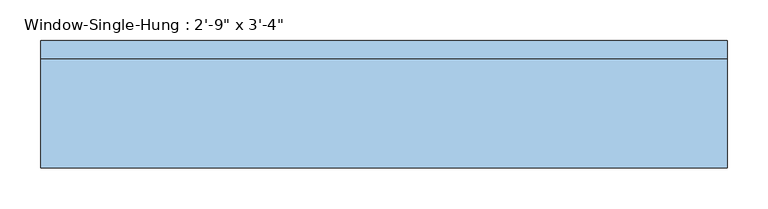
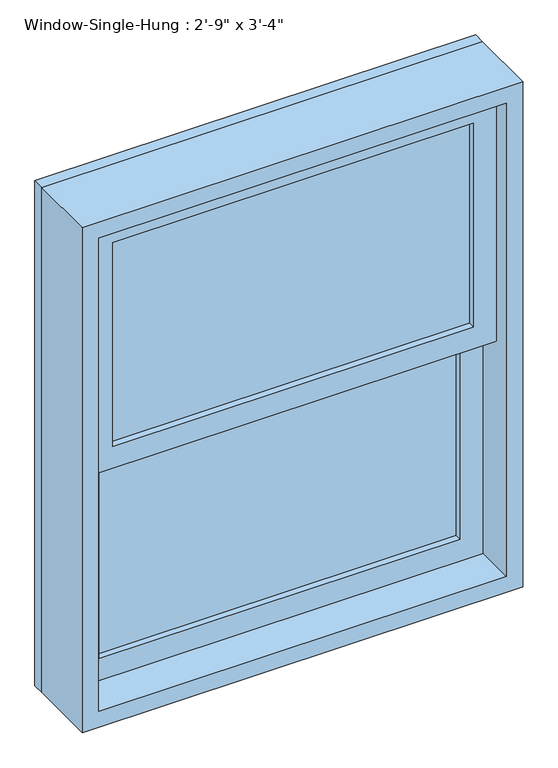
"""IFC4 building model written with IfcOpenShell, lengths in millimetres: window geometry."""

from ifc_helpers import new_model, si_unit, frame, origin, place, context, project, spatial, polyline, outline, extrude, source, transform, mapped, element, save


def window_d23c6517(model_context):
    return source(origin(), model_context, "Body", "SweptSolid", [
        extrude(outline(polyline([(342.9, 1.5875), (-342.9, 1.5875), (-342.9, 7.9375), (342.9, 7.9375), (342.9, 1.5875)])), frame((0.0, 0.0, 990.6), z_axis=(0.0, 0.0, 1.0), x_axis=(1.0, 0.0, 0.0)), (0.0, 0.0, 1.0), 409.575),
        extrude(outline(polyline([(-342.9, 14.2875), (-342.9, 20.6375), (342.9, 20.6375), (342.9, 14.2875), (-342.9, 14.2875)])), frame((0.0, 0.0, 990.6), z_axis=(0.0, 0.0, 1.0), x_axis=(1.0, 0.0, 0.0)), (0.0, 0.0, 1.0), 409.575),
        extrude(outline(polyline([(342.9, -42.8625), (-342.9, -42.8625), (-342.9, -36.5125), (342.9, -36.5125), (342.9, -42.8625)])), frame((0.0, 0.0, 1444.625), z_axis=(0.0, 0.0, 1.0), x_axis=(1.0, 0.0, 0.0)), (0.0, 0.0, 1.0), 409.575),
        extrude(outline(polyline([(-342.9, -30.1625), (-342.9, -23.8125), (342.9, -23.8125), (342.9, -30.1625), (-342.9, -30.1625)])), frame((0.0, 0.0, 1444.625), z_axis=(0.0, 0.0, 1.0), x_axis=(1.0, 0.0, 0.0)), (0.0, 0.0, 1.0), 409.575),
        extrude(outline(polyline([(1444.625, 387.35), (1444.625, -387.35), (946.15, -387.35), (946.15, 387.35), (1444.625, 387.35)]), holes=[polyline([(1400.175, -342.9), (1400.175, 342.9), (990.6, 342.9), (990.6, -342.9), (1400.175, -342.9)])]), frame((0.0, -11.1125, 0.0), z_axis=(0.0, 1.0, 0.0), x_axis=(0.0, 0.0, 1.0)), (0.0, 0.0, 1.0), 44.45),
        extrude(outline(polyline([(1898.65, 387.35), (1898.65, -387.35), (1400.175, -387.35), (1400.175, 387.35), (1898.65, 387.35)]), holes=[polyline([(1854.2, -342.9), (1854.2, 342.9), (1444.625, 342.9), (1444.625, -342.9), (1854.2, -342.9)])]), frame((0.0, -55.5625, 0.0), z_axis=(0.0, 1.0, 0.0), x_axis=(0.0, 0.0, 1.0)), (0.0, 0.0, 1.0), 44.45),
        extrude(outline(polyline([(1930.4, 419.1), (1930.4, -419.1), (914.4, -419.1), (914.4, 419.1), (1930.4, 419.1)]), holes=[polyline([(1898.65, -387.35), (1898.65, 387.35), (946.15, 387.35), (946.15, -387.35), (1898.65, -387.35)])]), frame((0.0, -87.3125, 0.0), z_axis=(0.0, 1.0, 0.0), x_axis=(0.0, 0.0, 1.0)), (0.0, 0.0, 1.0), 133.35),
        extrude(outline(polyline([(1930.4, 419.1), (1930.4, -419.1), (914.4, -419.1), (914.4, 419.1), (1930.4, 419.1)]), holes=[polyline([(1911.35, 400.05), (933.45, 400.05), (933.45, -400.05), (1911.35, -400.05), (1911.35, 400.05)])]), frame((0.0, 46.0375, 0.0), z_axis=(0.0, 1.0, 0.0), x_axis=(0.0, 0.0, 1.0)), (0.0, 0.0, 1.0), 22.225),
    ])


if __name__ == "__main__":
    model = new_model("IFC4")
    model_context = context("Model", 3, world=origin())
    ifc_project = project(units=[si_unit("LENGTHUNIT", "METRE", prefix="MILLI")], contexts=[model_context])
    site = spatial("IfcSite", under=ifc_project)
    building = spatial("IfcBuilding", under=site)
    placement = place(None, origin())
    window_shape = window_d23c6517(model_context)
    element("IfcWindow", 1, ObjectType="Window-Single-Hung : 2'-9\" x 3'-4\"", at=placement, inside=building, context=model_context, shape_type="MappedRepresentation", body=[
        mapped(window_shape, transform((0.0, 0.0, 0.0), x_axis=(1.0, 0.0, 0.0), y_axis=(0.0, 1.0, 0.0), z_axis=(0.0, 0.0, 1.0))),
    ])
    save(model, "model.ifc")

# Revit data of these elements
# Type "Window-Single-Hung : 2'-9\" x 3'-4\""
#   Type Mark = "22"
#   Fire Rating = "0.5h"
#   Construction Type Id = "DG-DR"
#   Assembly Code = "B2020100"
#   Analytic Construction = "Double glazing - domestic"
#   Wall Thickness [instance default] = 0' - 6"
#   Window Inset [instance default] = 0' - 0"
#   Visual Light Transmittance = 0.81
#   Thermal Resistance (R) = 0.319569 (m²·K)/W
#   Solar Heat Gain Coefficient = 0.76
#   Muntin Width = 2' - 3"
#   Muntin Height = 1' - 4 1/8"
#   Interior Wall Closure [instance default] = 0' - 1 1/2"
#   Rough Width = 2' - 9 1/2"
#   Rough Height = 3' - 4 1/2"
#   Frame Extension [instance default] = 0' - 1 1/4"
#   Exterior Wall Closure [instance default] = 0' - 0 1/2"
#   Extension Jamb [instance default] = 0' - 1 1/2"
#   Heat Transfer Coefficient (U) = 3.12929 W/(m²·K)
#   Height = 3' - 4"
#   Width = 2' - 9"
#   Top Muntin Visibility = yes
#   Indicator Visibility [instance default] = yes
#   Extension Jamb Visibility [instance default] = yes
#   Interior Trim Visibility [instance default] = yes
#   Exterior Trim Visibility [instance default] = yes
#   Bottom Muntin Visibility = yes
#   Muntin Pattern = Muntin Pattern_2x2 : Muntin Pattern_2x2
#   Interior Trim Material = Wood - Stained
#   Interior Trim = Trim-Window-Interior-Flat : Picture Frame
#   Exterior Trim Material = Clad - White
#   Exterior Trim = Trim-Window-Exterior-Flat : with Sill
#   Glass Panel Material = Glass
#   Exterior Frame Material = Clad - White
#   Interior Frame Material = Wood - Stained
#   Wall Closure = (empty or 0)
# Element 1 (IfcWindow, "Window-Single-Hung : 2'-9\" x 3'-4\"")
#   Wall Thickness = 0' - 5 3/8"
#   Extension Jamb = 0' - 0 7/8"
#   Materials on its faces: "Wood - Stained", "Glass", "Clad - White"
# Materials
#   "Wood - Stained": class "Wood", colour RGB 224 178 126, transparency 0, Cost = 0
#   "Clad - White": class "Wood", colour RGB 242 242 238, transparency 0, Cost = 0
#   "Glass": class "Glass", colour RGB 0 128 192, transparency 0.75, Description = "Soda Lime Glass", Cost = 0
